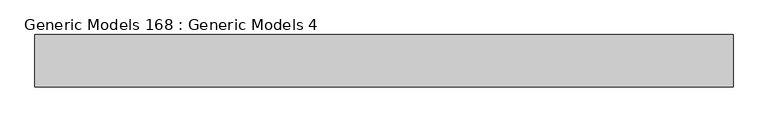
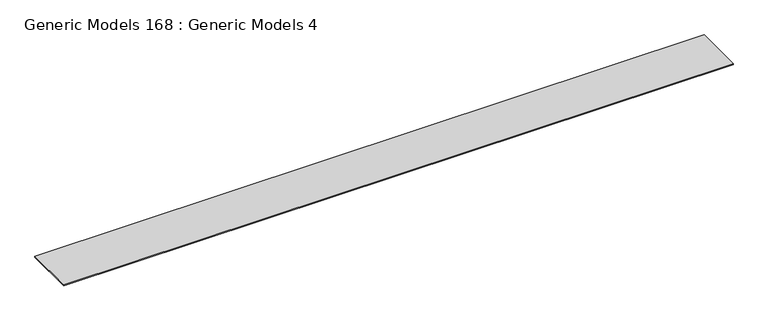
"""IFC4 building model written with IfcOpenShell, lengths in millimetres: proxy geometry, Generic Models 168 : Generic Models 4."""

from ifc_helpers import new_model, si_unit, frame, origin, place, context, project, spatial, polyline, outline, extrude, source, transform, mapped, element, save


def generic_models_168_generic_models_4_256463e9(model_context):
    return source(origin(), model_context, "Body", "SweptSolid", [
        extrude(outline(polyline([(-8342.1048025, -29686.8057997), (-8342.1048025, -30617.9735041), (-20795.7733045, -30617.9735041), (-20795.7733045, -29686.8057997), (-8342.1048025, -29686.8057997)])), frame((0.0, 0.0, 126809.246), z_axis=(0.0, 0.0, 1.0), x_axis=(1.0, 0.0, 0.0)), (0.0, 0.0, 1.0), 19.05),
    ])


if __name__ == "__main__":
    model = new_model("IFC4")
    model_context = context("Model", 3, world=origin())
    ifc_project = project(units=[si_unit("LENGTHUNIT", "METRE", prefix="MILLI")], contexts=[model_context])
    site = spatial("IfcSite", under=ifc_project)
    building = spatial("IfcBuilding", under=site)
    placement = place(None, origin())
    generic_models_168_generic_models_4_shape = generic_models_168_generic_models_4_256463e9(model_context)
    element("IfcBuildingElementProxy", 1, Name="Generic Models 168 : Generic Models 4", ObjectType="Generic Models 168 : Generic Models 4", at=placement, inside=building, context=model_context, shape_type="MappedRepresentation", body=[
        mapped(generic_models_168_generic_models_4_shape, transform((0.0, 0.0, 0.0), x_axis=(1.0, 0.0, 0.0), y_axis=(0.0, 1.0, 0.0), z_axis=(0.0, 0.0, 1.0))),
    ])
    save(model, "model.ifc")

# Revit data of these elements
# Element 1 (IfcBuildingElementProxy, "Generic Models 168 : Generic Models 4")
#   Materials on its faces: "_CDX PLYWOOD - SEE STRUCT DWGs"
# Materials
#   "_CDX PLYWOOD - SEE STRUCT DWGs": class "Generic", colour RGB 98 75 74, transparency 0, Cost = 0
